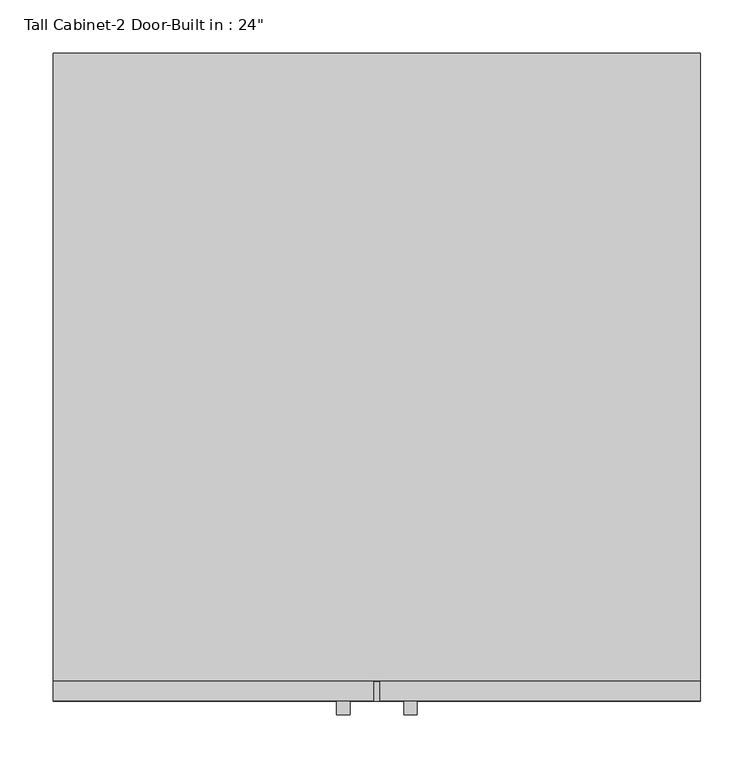
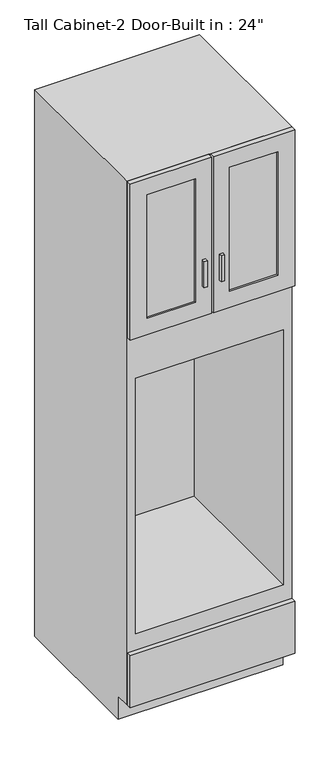
"""IFC4 building model written with IfcOpenShell, lengths in millimetres: furniture geometry."""

from ifc_helpers import new_model, si_unit, frame, origin, place, context, project, spatial, polyline, outline, extrude, faceted_brep, source, transform, mapped, element, save


def furniture_1eba2136(model_context):
    return source(origin(), model_context, "Body", "SolidModel", [
        faceted_brep([(323.5377049, -590.55, 90.4875), (323.5377049, -590.55, 2135.1875), (-286.0622951, -590.55, 2135.1875), (-286.0622951, -590.55, 90.4875), (-267.0122951, -590.55, 2116.1375), (304.4877049, -590.55, 2116.1375), (304.4877049, -590.55, 1525.5875), (-267.0122951, -590.55, 1525.5875), (291.7877049, -590.55, 357.1875), (-254.3122951, -590.55, 357.1875), (-254.3122951, -590.55, 1354.1375), (291.7877049, -590.55, 1354.1375), (-286.0622951, 0.0, 2135.1875), (323.5377049, 0.0, 2135.1875), (323.5377049, 0.0, 0.0), (-286.0622951, 0.0, 0.0), (323.5377049, -533.4, 90.4875), (323.5377049, -533.4, 0.0), (-286.0622951, -533.4, 0.0), (-286.0622951, -533.4, 90.4875), (304.4877049, -19.05, 2116.1375), (304.4877049, -19.05, 1525.5875), (-267.0122951, -19.05, 1525.5875), (-267.0122951, -19.05, 2116.1375), (291.7877049, -19.05, 357.1875), (-254.3122951, -19.05, 357.1875), (-254.3122951, -19.05, 1354.1375), (291.7877049, -19.05, 1354.1375)], [[[0, 1, 2, 3], [4, 5, 6, 7], [8, 9, 10, 11]], [[12, 13, 14, 15]], [[1, 0, 16, 17, 14, 13]], [[2, 1, 13, 12]], [[3, 2, 12, 15, 18, 19]], [[0, 3, 19, 16]], [[6, 5, 20, 21]], [[4, 7, 22, 23]], [[5, 4, 23, 20]], [[14, 17, 18, 15]], [[18, 17, 16, 19]], [[7, 6, 21, 22]], [[9, 8, 24, 25]], [[10, 9, 25, 26]], [[11, 10, 26, 27]], [[8, 11, 27, 24]], [[21, 20, 23, 22]], [[25, 24, 27, 26]]]),
        extrude(outline(polyline([(323.5377049, -609.6), (-286.0622951, -609.6), (-286.0622951, -590.55), (323.5377049, -590.55), (323.5377049, -609.6)])), frame((0.0, 0.0, 90.4875), z_axis=(0.0, 0.0, 1.0), x_axis=(1.0, 0.0, 0.0)), (0.0, 0.0, 1.0), 203.2),
        extrude(outline(polyline([(2135.1875, 15.5627049), (2135.1875, -286.0622951), (1525.5875, -286.0622951), (1525.5875, 15.5627049), (2135.1875, 15.5627049)]), holes=[polyline([(2071.6875, -44.7622951), (1589.0875, -44.7622951), (1589.0875, -222.5622951), (2071.6875, -222.5622951), (2071.6875, -44.7622951)])]), frame((0.0, -609.6, 0.0), z_axis=(0.0, 1.0, 0.0), x_axis=(0.0, 0.0, 1.0)), (0.0, 0.0, 1.0), 19.05),
        extrude(outline(polyline([(2135.1875, 21.9127049), (1525.5875, 21.9127049), (1525.5875, 323.5377049), (2135.1875, 323.5377049), (2135.1875, 21.9127049)]), holes=[polyline([(2071.6875, 260.0377049), (1589.0875, 260.0377049), (1589.0875, 82.2377049), (2071.6875, 82.2377049), (2071.6875, 260.0377049)])]), frame((0.0, -609.6, 0.0), z_axis=(0.0, 1.0, 0.0), x_axis=(0.0, 0.0, 1.0)), (0.0, 0.0, 1.0), 19.05),
        extrude(outline(polyline([(323.5377049, -609.6), (-286.0622951, -609.6), (-286.0622951, -590.55), (323.5377049, -590.55), (323.5377049, -609.6)])), frame((0.0, 0.0, 90.4875), z_axis=(0.0, 0.0, 1.0), x_axis=(1.0, 0.0, 0.0)), (0.0, 0.0, 1.0), 203.2),
        extrude(outline(polyline([(-6.6622951, -622.3), (-19.1945267, -622.3), (-19.1945267, -609.6), (-6.6622951, -609.6), (-6.6622951, -622.3)])), frame((0.0, 0.0, 1645.6417867), z_axis=(0.0, 0.0, 1.0), x_axis=(1.0, 0.0, 0.0)), (0.0, 0.0, 1.0), 101.6),
        extrude(outline(polyline([(56.6699365, -622.3), (44.1377049, -622.3), (44.1377049, -609.6), (56.6699365, -609.6), (56.6699365, -622.3)])), frame((0.0, 0.0, 1645.6417867), z_axis=(0.0, 0.0, 1.0), x_axis=(1.0, 0.0, 0.0)), (0.0, 0.0, 1.0), 101.6),
        extrude(outline(polyline([(-44.7622951, -603.25), (-222.5622951, -603.25), (-222.5622951, -596.9), (-44.7622951, -596.9), (-44.7622951, -603.25)])), frame((0.0, 0.0, 1589.0875), z_axis=(0.0, 0.0, 1.0), x_axis=(1.0, 0.0, 0.0)), (0.0, 0.0, 1.0), 482.6),
        extrude(outline(polyline([(260.0377049, -603.25), (82.2377049, -603.25), (82.2377049, -596.9), (260.0377049, -596.9), (260.0377049, -603.25)])), frame((0.0, 0.0, 1589.0875), z_axis=(0.0, 0.0, 1.0), x_axis=(1.0, 0.0, 0.0)), (0.0, 0.0, 1.0), 482.6),
    ])


if __name__ == "__main__":
    model = new_model("IFC4")
    model_context = context("Model", 3, world=origin())
    ifc_project = project(units=[si_unit("LENGTHUNIT", "METRE", prefix="MILLI")], contexts=[model_context])
    site = spatial("IfcSite", under=ifc_project)
    building = spatial("IfcBuilding", under=site)
    placement = place(None, origin())
    furniture_shape = furniture_1eba2136(model_context)
    element("IfcFurniture", 1, ObjectType="Tall Cabinet-2 Door-Built in : 24\"", at=placement, inside=building, context=model_context, shape_type="MappedRepresentation", body=[
        mapped(furniture_shape, transform((0.0, 0.0, 0.0), x_axis=(1.0, 0.0, 0.0), y_axis=(0.0, 1.0, 0.0), z_axis=(0.0, 0.0, 1.0))),
    ])
    save(model, "model.ifc")

# Revit data of these elements
# Project information
#   Project Issue Date = "Issue Date"
#   Project Status = "Project Status"
#   Client Name = "Owner"
#   Project Address = "Enter address here"
#   Project Name = "Project Name"
#   Project Number = "Project Number"
# Type "Tall Cabinet-2 Door-Built in : 24\""
#   Assembly Code = "C1030410"
#   Type Comments = "21.5\"w 39.75\"h built-in"
#   Height = 7' - 0"
#   Depth = 2' - 0"
#   Height-Base of Built-in = 1' - 2"
#   Height-Built-in = 3' - 3 1/4"
#   Height-Upper Cabinet = 2' - 0"
#   Toe Depth = 0' - 3"
#   Toe Height = 0' - 3 1/2"
#   Width = 2' - 0"
#   Cabinet Material = none
#   Door/Drawer Material = none
#   Handle Material = Cabinets - Handles
#   Panel Material = Glass
# Element 1 (IfcFurniture, "Tall Cabinet-2 Door-Built in : 24\"")
#   Materials on its faces: "Cabinets", "Cabinets - Handles", "Glass"
# Materials
#   "Cabinets - Handles": class "Metal", colour RGB 57 57 57, transparency 0
#   "Glass": class "Glass", colour RGB 0 128 192, transparency 0.75, Description = "Soda Lime Glass", Cost = 0
#   "Cabinets": class "Miscellaneous", colour RGB 249 249 249, transparency 0
